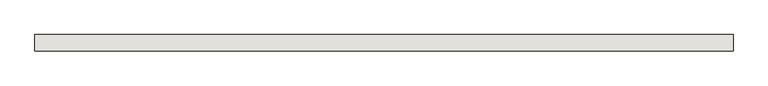
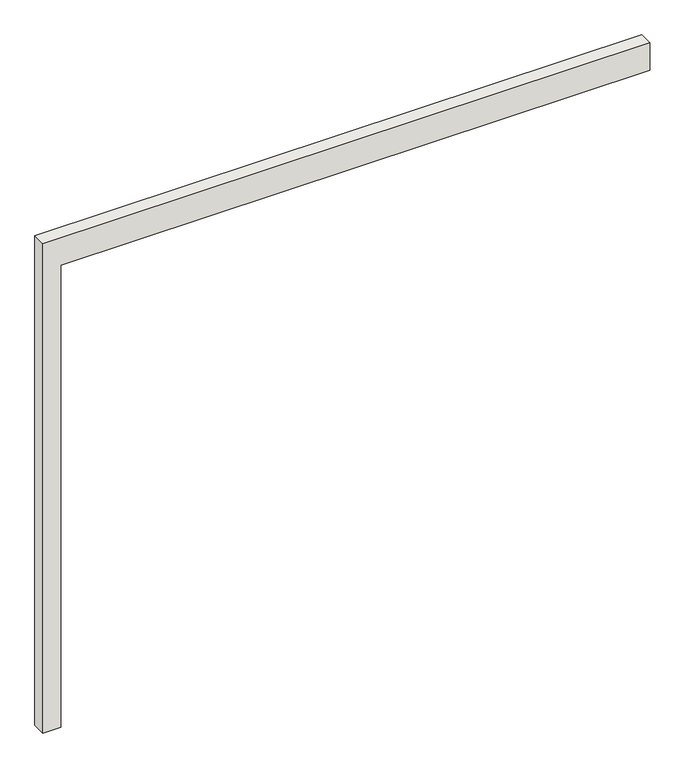
"""IFC4 building model written with IfcOpenShell, lengths in millimetres: wall geometry, 0_3d_modell."""

from ifc_helpers import new_model, si_unit, frame, origin, place, context, project, spatial, polyline, outline, extrude, source, transform, mapped, element, save


def wall_42740fb9(model_context):
    return source(origin(), model_context, "Body", "SweptSolid", [
        extrude(outline(polyline([(0.0, 100.0), (2720.0, 100.0), (2720.0, 3378.0), (2880.0, 3378.0), (2880.0, 0.0), (0.0, 0.0), (0.0, 100.0)])), frame((0.0, 0.0, 0.0), z_axis=(0.0, 1.0, 0.0), x_axis=(0.0, 0.0, 1.0)), (0.0, 0.0, 1.0), 78.0),
    ])


if __name__ == "__main__":
    model = new_model("IFC4")
    model_context = context("Model", 3, world=origin())
    ifc_project = project(units=[si_unit("LENGTHUNIT", "METRE", prefix="MILLI")], contexts=[model_context])
    site = spatial("IfcSite", under=ifc_project)
    building = spatial("IfcBuilding", under=site)
    placement = place(None, origin())
    wall_shape = wall_42740fb9(model_context)
    element("IfcWall", 1, ObjectType="0_3d_modell", at=placement, inside=building, context=model_context, shape_type="MappedRepresentation", body=[
        mapped(wall_shape, transform((0.0, 0.0, 0.0), x_axis=(1.0, 0.0, 0.0), y_axis=(0.0, 1.0, 0.0), z_axis=(0.0, 0.0, 1.0))),
    ])
    save(model, "model.ifc")

# Revit data of these elements
# Element 1 (IfcWall, "0_3d_modell")
#   Materials on its faces: "glas"
# Materials
#   "glas": class "Unassigned", colour RGB 250 253 254, transparency 0.95
